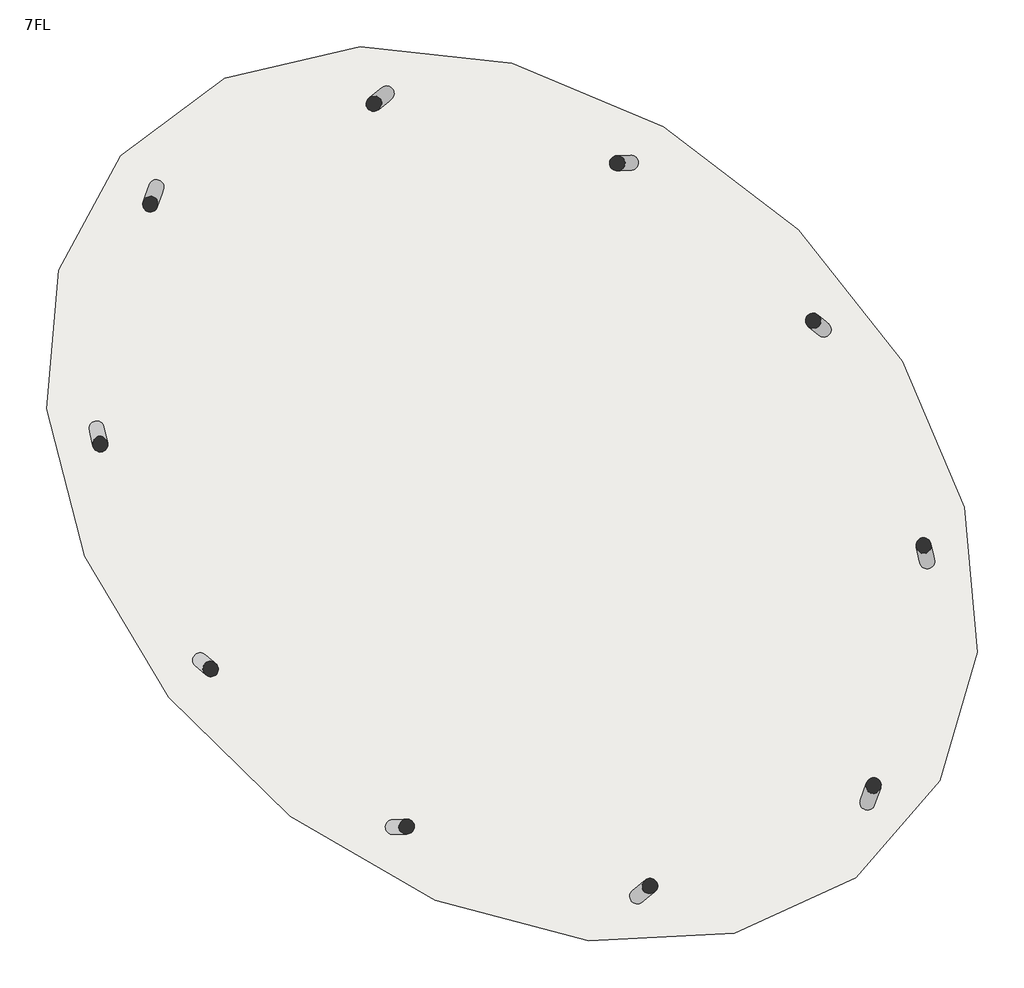
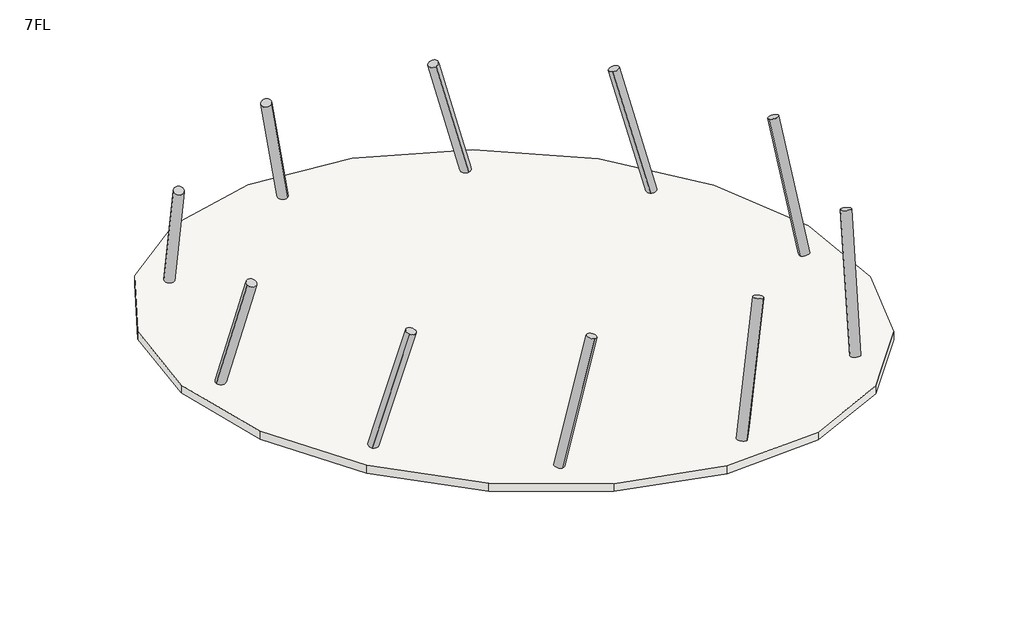
# One storey: 10 columns, 1 slab.
"""IFC4 building model written with IfcOpenShell, lengths in millimetres."""

from ifc_helpers import new_model, si_unit, point, frame, frame_2d, origin, place, context, project, spatial, polyline, circle_curve, trimmed, segment, composite_curve, outline, extrude, element, save

model = new_model("IFC4")

# Units and contexts
model_context = context("Model", 3, world=origin())
ifc_project = project(units=[si_unit("LENGTHUNIT", "METRE", prefix="MILLI")], contexts=[model_context])

# Site, building, storey
site = spatial("IfcSite", under=ifc_project)
building = spatial("IfcBuilding", under=site)
storey = spatial("IfcBuildingStorey", under=building, Name="7FL", Elevation=27000.0)

# Columns
placement = place(None, origin())
element("IfcColumn", 1, ObjectType="コンクリート-円形-柱 : 750", at=placement, inside=storey, context=model_context, shape_type="SweptSolid", body=[
    extrude(outline(composite_curve([segment(trimmed(circle_curve(frame_2d((0.0, -175.0)), 175.0), [point((0.0, -350.0000001))], [point((0.0, 0.0))], False, "CARTESIAN"), True, "CONTINUOUS"), segment(trimmed(circle_curve(frame_2d((0.0, -175.0)), 175.0), [point((0.0, 0.0))], [point((0.0, -350.0000001))], False, "CARTESIAN"), True, "CONTINUOUS")], self_intersect=False)), frame((-8101.9911662, 7105.4476808, 27000.0), z_axis=(-0.11108929791393216, -0.31607244423933784, 0.9422087761645825), x_axis=(-0.31242117778064243, -0.8889040361904746, -0.3350263006368899)), (0.0, 0.0, 1.0), 4776.0115527),
])
element("IfcColumn", 2, ObjectType="コンクリート-円形-柱 : 750", at=placement, inside=storey, context=model_context, shape_type="SweptSolid", body=[
    extrude(outline(composite_curve([segment(trimmed(circle_curve(frame_2d((0.0, -175.0)), 175.0), [point((0.0, -350.0000001))], [point((0.0, 0.0))], False, "CARTESIAN"), True, "CONTINUOUS"), segment(trimmed(circle_curve(frame_2d((0.0, -175.0)), 175.0), [point((0.0, 0.0))], [point((0.0, -350.0000001))], False, "CARTESIAN"), True, "CONTINUOUS")], self_intersect=False)), frame((-9488.3111438, 1589.8784362, 27000.0), z_axis=(0.0663013781536146, -0.29532584628371034, 0.9530932649912818), x_axis=(0.20877517818073227, -0.9299460719565116, -0.3026767718677109)), (0.0, 0.0, 1.0), 4721.4686802),
])
element("IfcColumn", 3, ObjectType="コンクリート-円形-柱 : 750", at=placement, inside=storey, context=model_context, shape_type="SweptSolid", body=[
    extrude(outline(composite_curve([segment(trimmed(circle_curve(frame_2d((0.0, -175.0)), 175.0), [point((0.0, -350.0))], [point((0.0, 0.0))], False, "CARTESIAN"), True, "CONTINUOUS"), segment(trimmed(circle_curve(frame_2d((0.0, -175.0)), 175.0), [point((0.0, 0.0))], [point((0.0, -350.0))], False, "CARTESIAN"), True, "CONTINUOUS")], self_intersect=False)), frame((-7140.0684248, -3709.5068437, 27000.0), z_axis=(0.1974132787427203, -0.16585051342227883, 0.9661892177899811), x_axis=(0.7397726720508109, -0.6214965794438607, -0.2578340462902145)), (0.0, 0.0, 1.0), 4657.4727984),
])
element("IfcColumn", 4, ObjectType="コンクリート-円形-柱 : 750", at=placement, inside=storey, context=model_context, shape_type="SweptSolid", body=[
    extrude(outline(composite_curve([segment(trimmed(circle_curve(frame_2d((0.0, -175.0)), 175.0), [point((-1e-07, -350.0))], [point((0.0, 0.0))], False, "CARTESIAN"), True, "CONTINUOUS"), segment(trimmed(circle_curve(frame_2d((0.0, -175.0)), 175.0), [point((0.0, 0.0))], [point((-1e-07, -350.0))], False, "CARTESIAN"), True, "CONTINUOUS")], self_intersect=False)), frame((-2779.1005081, -7550.9370791, 27000.0), z_axis=(0.2585133759612969, 0.010174404300097226, 0.9659540961899957), x_axis=(0.9652068318594687, 0.03798799386699609, -0.25871351733871323)), (0.0, 0.0, 1.0), 4658.6064694),
])
element("IfcColumn", 5, ObjectType="コンクリート-円形-柱 : 750", at=placement, inside=storey, context=model_context, shape_type="SweptSolid", body=[
    extrude(outline(composite_curve([segment(trimmed(circle_curve(frame_2d((0.0, -175.0)), 175.0), [point((0.0, -350.0))], [point((0.0, 0.0))], False, "CARTESIAN"), True, "CONTINUOUS"), segment(trimmed(circle_curve(frame_2d((0.0, -175.0)), 175.0), [point((0.0, 0.0))], [point((0.0, -350.0))], False, "CARTESIAN"), True, "CONTINUOUS")], self_intersect=False)), frame((2800.1880734, -9203.9866295, 27000.0), z_axis=(0.23607455187263401, 0.1913443790107675, 0.9527098900395223), x_axis=(0.7401262758384448, 0.5998910154291638, -0.3038813344397468)), (0.0, 0.0, 1.0), 4723.3686194),
])
element("IfcColumn", 6, ObjectType="コンクリート-円形-柱 : 750", at=placement, inside=storey, context=model_context, shape_type="SweptSolid", body=[
    extrude(outline(composite_curve([segment(trimmed(circle_curve(frame_2d((0.0, -175.0)), 175.0), [point((1e-07, -350.0))], [point((0.0, 0.0))], False, "CARTESIAN"), True, "CONTINUOUS"), segment(trimmed(circle_curve(frame_2d((0.0, -175.0)), 175.0), [point((0.0, 0.0))], [point((1e-07, -350.0))], False, "CARTESIAN"), True, "CONTINUOUS")], self_intersect=False)), frame((8101.9912014, -7105.4476678, 27000.0), z_axis=(0.11108929725860742, 0.3160724452716469, 0.9422087758955499), x_axis=(0.31242117514287665, 0.8889040368323988, -0.33502630139350176)), (0.0, 0.0, 1.0), 4776.0115527),
])
element("IfcColumn", 7, ObjectType="コンクリート-円形-柱 : 750", at=placement, inside=storey, context=model_context, shape_type="SweptSolid", body=[
    extrude(outline(composite_curve([segment(trimmed(circle_curve(frame_2d((0.0, -175.0)), 175.0), [point((0.0, -350.0))], [point((0.0, 0.0))], False, "CARTESIAN"), True, "CONTINUOUS"), segment(trimmed(circle_curve(frame_2d((0.0, -175.0)), 175.0), [point((0.0, 0.0))], [point((0.0, -350.0))], False, "CARTESIAN"), True, "CONTINUOUS")], self_intersect=False)), frame((9488.3111375, -1589.8784158, 27000.0), z_axis=(-0.0663013802162775, 0.2953258459577328, 0.9530932649488014), x_axis=(-0.2087751845742411, 0.9299460704776152, -0.30267677200147675)), (0.0, 0.0, 1.0), 4721.4686802),
])
element("IfcColumn", 8, ObjectType="コンクリート-円形-柱 : 750", at=placement, inside=storey, context=model_context, shape_type="SweptSolid", body=[
    extrude(outline(composite_curve([segment(trimmed(circle_curve(frame_2d((0.0, -175.0000001)), 175.0), [point((-1e-07, -350.0))], [point((0.0, 0.0))], False, "CARTESIAN"), True, "CONTINUOUS"), segment(trimmed(circle_curve(frame_2d((0.0, -175.0000001)), 175.0), [point((0.0, 0.0))], [point((-1e-07, -350.0))], False, "CARTESIAN"), True, "CONTINUOUS")], self_intersect=False)), frame((7140.0684006, 3709.5068517, 27000.0), z_axis=(-0.19741327939264486, 0.16585051275612087, 0.9661892177715363), x_axis=(-0.7397726742738567, 0.6214965767690758, -0.25783404635933305)), (0.0, 0.0, 1.0), 4657.4727984),
])
element("IfcColumn", 9, ObjectType="コンクリート-円形-柱 : 750", at=placement, inside=storey, context=model_context, shape_type="SweptSolid", body=[
    extrude(outline(composite_curve([segment(trimmed(circle_curve(frame_2d((0.0, -175.0)), 175.0), [point((-1e-07, -350.0))], [point((0.0, 0.0))], False, "CARTESIAN"), True, "CONTINUOUS"), segment(trimmed(circle_curve(frame_2d((0.0, -175.0)), 175.0), [point((0.0, 0.0))], [point((-1e-07, -350.0))], False, "CARTESIAN"), True, "CONTINUOUS")], self_intersect=False)), frame((2779.1005536, 7550.9370567, 27000.0), z_axis=(-0.25851337771301813, -0.010174402063420553, 0.9659540957447503), x_axis=(-0.9652068317528497, -0.03798798525434792, -0.2587135190011178)), (0.0, 0.0, 1.0), 4658.6064694),
])
element("IfcColumn", 10, ObjectType="コンクリート-円形-柱 : 750", at=placement, inside=storey, context=model_context, shape_type="SweptSolid", body=[
    extrude(outline(composite_curve([segment(trimmed(circle_curve(frame_2d((0.0, -175.0)), 175.0), [point((0.0, -350.0))], [point((0.0, 0.0))], False, "CARTESIAN"), True, "CONTINUOUS"), segment(trimmed(circle_curve(frame_2d((0.0, -175.0)), 175.0), [point((0.0, 0.0))], [point((0.0, -350.0))], False, "CARTESIAN"), True, "CONTINUOUS")], self_intersect=False)), frame((-2800.1879936, 9203.9866345, 27000.0), z_axis=(-0.23607455347688813, -0.19134437564637777, 0.9527098903177115), x_axis=(-0.7401262832083332, -0.5998910067782347, -0.3038813335675856)), (0.0, 0.0, 1.0), 4723.3686194),
])

# Slab
element("IfcSlab", 11, ObjectType="一般 300 mm", at=placement, inside=storey, context=model_context, shape_type="SweptSolid", body=[
    extrude(outline(polyline([(-10823.0158083, 2005.0174013), (-10535.6906394, 5226.8245056), (-9100.263229, 7885.4229754), (-6673.0080781, 9684.5978157), (-3524.8849596, 10427.5093857), (-0.8045627, 10039.2581476), (3519.7972118, 8566.6384187), (6659.4752244, 6170.2590168), (9081.098151, 3108.0253246), (10523.2925046, -291.8678958), (10827.4867995, -3665.1205394), (9954.7726107, -6646.88205), (7995.9382136, -8907.4974181), (5168.7269365, -10195.6775707), (1786.5177728, -10374.64343), (-1784.0150983, -9430.9838116), (-5159.7125355, -7469.8107787), (-7978.5230253, -4703.1305154), (-9937.1874762, -1427.9390261), (-10823.0158083, 2005.0174013)])), frame((0.0, 0.0, 26700.0), z_axis=(0.0, 0.0, 1.0), x_axis=(1.0, 0.0, 0.0)), (0.0, 0.0, 1.0), 300.0),
])

save(model, "model.ifc")

# Revit data of these elements
# Type "コンクリート-円形-柱 : 750"
#   Keynote = "03310.Q1"
#   R = 350 mm
#   Structural Material [instance default] = コンクリート - 現場打ち
# Type "一般 300 mm"
#   Function = 0
#   Layers, outside or top first: 300 mm no material (function 1)
# Elements 1, 2, 3, 4, 5, 6, 7, 8, 9, 10 (IfcColumn, "コンクリート-円形-柱 : 750")
#   Structural Material = コンクリート - 現場打ち
#   Phase Created = 新しい建設
#   Materials on its faces: "コンクリート - 現場打ち"
# Element 11 (IfcSlab, "一般 300 mm")
#   Height Offset From Level = 0 mm
#   Phase Created = 新しい建設
# Materials
#   "コンクリート - 現場打ち": class "コンクリート", colour RGB 192 192 192, transparency 0
